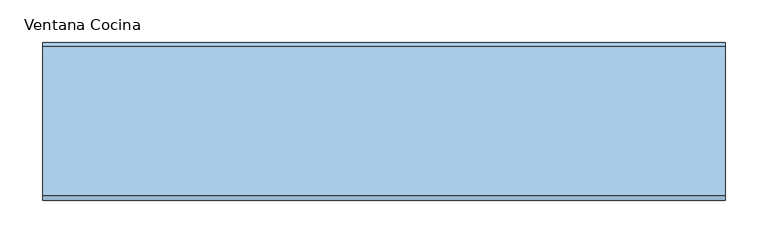
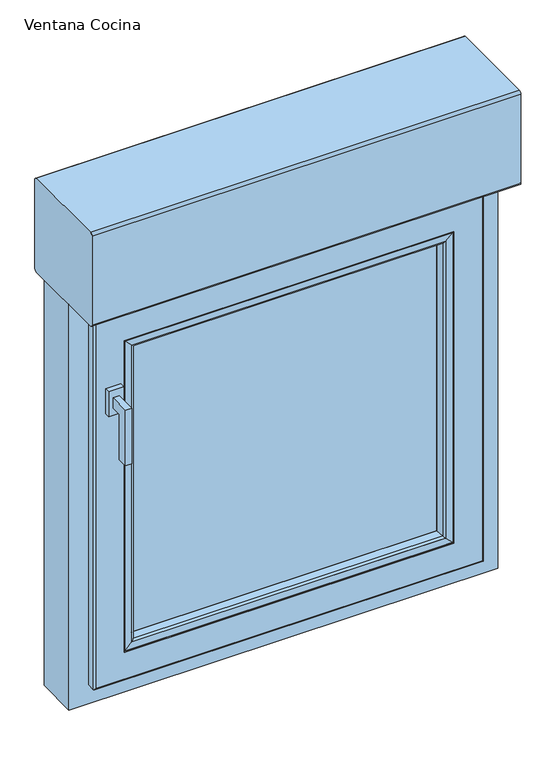
"""IFC4 building model written with IfcOpenShell, lengths in millimetres: window geometry, 2019_ES_Ventana_Replus_re80pvc301_10100_box_1-Hoja_con-Compacto : Ventana Cocina."""

from ifc_helpers import new_model, si_unit, point, frame, frame_2d, origin, place, context, project, spatial, polyline, circle_curve, ellipse_curve, trimmed, segment, composite_curve, outline, extrude, source, transform, mapped, element, save
from ifc_brep_helpers import plane_surface, cylinder_surface, advanced_brep


def ventana_cocina_321dc98e(model_context):
    return source(origin(), model_context, "Body", "SolidModel", [
        extrude(outline(composite_curve([segment(polyline([(55.0, 1610.0), (-120.0, 1610.0)]), True, "CONTINUOUS"), segment(trimmed(circle_curve(frame_2d((-120.0, 1615.0)), 5.0), [point((-120.0, 1610.0))], [point((-125.0, 1615.0))], False, "CARTESIAN"), True, "CONTINUOUS"), segment(polyline([(-125.0, 1615.0), (-125.0, 1790.0)]), True, "CONTINUOUS"), segment(trimmed(circle_curve(frame_2d((-120.0, 1790.0)), 5.0), [point((-125.0, 1790.0))], [point((-120.0, 1795.0))], False, "CARTESIAN"), True, "CONTINUOUS"), segment(polyline([(-120.0, 1795.0), (55.0, 1795.0)]), True, "CONTINUOUS"), segment(trimmed(circle_curve(frame_2d((55.0, 1790.0)), 5.0), [point((55.0, 1795.0))], [point((60.0, 1790.0))], False, "CARTESIAN"), True, "CONTINUOUS"), segment(polyline([(60.0, 1790.0), (60.0, 1615.0)]), True, "CONTINUOUS"), segment(trimmed(circle_curve(frame_2d((55.0, 1615.0)), 5.0), [point((60.0, 1615.0))], [point((55.0, 1610.0))], False, "CARTESIAN"), True, "CONTINUOUS")], self_intersect=False)), frame((-400.0, 0.0, 0.0), z_axis=(1.0, 0.0, 0.0), x_axis=(0.0, 1.0, 0.0)), (0.0, 0.0, 1.0), 800.0),
        extrude(outline(polyline([(-78.4999991, 1420.0), (-78.4999991, 1400.0), (-98.4999991, 1400.0), (-98.4999991, 1310.0), (-118.4999991, 1310.0), (-118.4999991, 1420.0), (-78.4999991, 1420.0)])), frame((-334.1999993, 0.0, 0.0), z_axis=(1.0, 0.0, 0.0), x_axis=(0.0, 1.0, 0.0)), (0.0, 0.0, 1.0), 12.0),
        extrude(outline(polyline([(-313.9687607, -78.4999991), (-342.4312378, -78.4999991), (-342.4312378, -68.4999991), (-313.9687607, -68.4999991), (-313.9687607, -78.4999991)])), frame((0.0, 0.0, 1385.217127), z_axis=(0.0, 0.0, 1.0), x_axis=(1.0, 0.0, 0.0)), (0.0, 0.0, 1.0), 49.565746),
        extrude(outline(polyline([(1507.2, 297.1999993), (1507.2, -297.1999993), (909.8, -297.1999993), (909.8, 297.1999993), (1507.2, 297.1999993)]), holes=[polyline([(917.8, 289.1999993), (917.8, -289.1999993), (1499.2, -289.1999993), (1499.2, 289.1999993), (917.8, 289.1999993)])]), frame((0.0, -26.9999999, 0.0), z_axis=(0.0, 1.0, 0.0), x_axis=(0.0, 0.0, 1.0)), (0.0, 0.0, 1.0), 16.0),
        extrude(outline(polyline([(1507.1868066, 297.1868058), (1507.1868066, -297.1868058), (909.8131934, -297.1868058), (909.8131934, 297.1868058), (1507.1868066, 297.1868058)]), holes=[polyline([(917.8, 289.1999993), (917.8, -289.1999993), (1499.2, -289.1999993), (1499.2, 289.1999993), (917.8, 289.1999993)])]), frame((0.0, -47.0000001, 0.0), z_axis=(0.0, 1.0, 0.0), x_axis=(0.0, 0.0, 1.0)), (0.0, 0.0, 1.0), 16.0),
        extrude(outline(polyline([(297.1999993, -6.9999997), (297.1999993, -10.9999999), (-297.1999993, -10.9999999), (-297.1999993, -6.9999997), (297.1999993, -6.9999997)])), frame((0.0, 0.0, 903.7946451), z_axis=(0.0, 0.0, 1.0), x_axis=(1.0, 0.0, 0.0)), (0.0, 0.0, 1.0), 609.4053549),
        extrude(outline(polyline([(297.1999993, -26.9999999), (297.1999993, -31.0000001), (-297.1999993, -31.0000001), (-297.1999993, -26.9999999), (297.1999993, -26.9999999)])), frame((0.0, 0.0, 903.7946451), z_axis=(0.0, 0.0, 1.0), x_axis=(1.0, 0.0, 0.0)), (0.0, 0.0, 1.0), 609.4053549),
        extrude(outline(polyline([(297.1999993, -47.0000001), (297.1999993, -51.0000003), (-297.1999993, -51.0000003), (-297.1999993, -47.0000001), (297.1999993, -47.0000001)])), frame((0.0, 0.0, 903.7946451), z_axis=(0.0, 0.0, 1.0), x_axis=(1.0, 0.0, 0.0)), (0.0, 0.0, 1.0), 609.4053549),
        advanced_brep(
        [(287.2913171, 9.2764571, 1497.2913178), (290.1890946, 11.5, 1500.1890953), (290.1890946, 11.5, 919.8109047), (287.2913171, 9.2764571, 922.7086822), (330.1999993, 11.5, 879.8), (-330.1999993, 11.5, 879.8), (-330.1999993, 11.5, 1540.2), (330.1999993, 11.5, 1540.2), (-290.1890946, 11.5, 1500.1890953), (-290.1890946, 11.5, 919.8109047), (-287.2913171, 9.2764571, 922.7086822), (284.1757968, -2.3508228, 1494.1757976), (284.1757968, -2.3508228, 925.8242024), (-284.1757968, -2.3508228, 925.8242024), (284.6739305, -3.0000033, 1494.6739313), (284.6739305, -3.0000033, 925.3260687), (-284.6739305, -3.0000033, 925.3260687), (291.1999993, -3.0000033, 1501.2), (-291.1999993, -3.0000033, 1501.2), (-291.1999993, -3.0000033, 918.8), (291.1999993, -3.0000033, 918.8), (-284.6739305, -3.0000033, 1494.6739313), (291.1999993, -6.9999997, 1501.2), (291.1999993, -6.9999997, 918.8), (-291.1999993, -6.9999997, 918.8), (311.8162192, -6.9999997, 1521.8162199), (-311.8162192, -6.9999997, 1521.8162199), (-311.8162192, -6.9999997, 898.1837801), (311.8162192, -6.9999997, 898.1837801), (-291.1999993, -6.9999997, 1501.2), (309.1999993, -25.6153717, 1519.2), (309.1999993, -25.6153717, 900.8), (-309.1999993, -25.6153717, 900.8), (309.1999993, -56.4999995, 1519.2), (309.1999993, -56.4999995, 900.8), (-309.1999993, -56.4999995, 900.8), (-309.1999993, -56.4999995, 1519.2), (297.1999993, -56.4999995, 1507.2), (-297.1999993, -56.4999995, 1507.2), (-297.1999993, -56.4999995, 912.8), (297.1999993, -56.4999995, 912.8), (297.1999993, -51.0000003, 1507.2), (297.1999993, -51.0000003, 912.8), (-297.1999993, -51.0000003, 912.8), (-297.1999993, -51.0000003, 1507.2), (286.007687, -51.0000003, 1496.0076877), (-286.007687, -51.0000003, 1496.0076877), (-286.007687, -51.0000003, 923.9923123), (286.007687, -51.0000003, 923.9923123), (285.4940999, -51.6693201, 1495.4941006), (285.4940999, -51.6693201, 924.5058994), (-285.4940999, -51.6693201, 924.5058994), (288.8993918, -64.3780426, 1498.8993925), (288.8993918, -64.3780426, 921.1006075), (-288.8993918, -64.3780426, 921.1006075), (292.6234971, -67.3403297, 1502.6234978), (292.6234971, -67.3403297, 917.3765022), (-292.6234971, -67.3403297, 917.3765022), (305.6488427, -67.7951848, 1515.6488434), (305.6488427, -67.7951848, 904.3511566), (-305.6488427, -67.7951848, 904.3511566), (306.1999993, -67.2629391, 1516.2), (306.1999993, -67.2629391, 903.8), (-306.1999993, -67.2629391, 903.8), (307.4370593, -68.4999991, 1517.43706), (307.4370593, -68.4999991, 902.56294), (-307.4370593, -68.4999991, 902.56294), (360.1999993, -68.4999991, 1570.2), (-360.1999993, -68.4999991, 1570.2), (-360.1999993, -68.4999991, 849.8), (360.1999993, -68.4999991, 849.8), (-307.4370593, -68.4999991, 1517.43706), (363.1999993, -65.4999991, 1573.2), (363.1999993, -65.4999991, 846.8), (-363.1999993, -65.4999991, 846.8), (363.1999993, -50.0, 1573.2), (363.1999993, -50.0, 846.8), (-363.1999993, -50.0, 846.8), (-363.1999993, -50.0, 1573.2), (343.1999993, -50.0, 1553.2), (-343.1999993, -50.0, 1553.2), (-343.1999993, -50.0, 866.8), (343.1999993, -50.0, 866.8), (343.1999993, -11.9999991, 866.8), (343.1999993, -11.9999991, 1553.2), (-343.1999993, -11.9999991, 866.8), (-343.1999993, -11.9999991, 1553.2), (330.1999993, -11.9999991, 1540.2), (-330.1999993, -11.9999991, 1540.2), (-330.1999993, -11.9999991, 879.8), (330.1999993, -11.9999991, 879.8), (-287.2913171, 9.2764571, 1497.2913178), (-284.1757968, -2.3508228, 1494.1757976), (-309.1999993, -25.6153717, 1519.2), (-285.4940999, -51.6693201, 1495.4941006), (-288.8993918, -64.3780426, 1498.8993925), (-292.6234971, -67.3403297, 1502.6234978), (-305.6488427, -67.7951848, 1515.6488434), (-306.1999993, -67.2629391, 1516.2), (-363.1999993, -65.4999991, 1573.2)],
        [
            (0, 1, ellipse_curve(frame((290.1890946, 8.5, 1500.1890953), z_axis=(0.7071067811865475, 0.0, -0.7071067811865475), x_axis=(0.7071067811865474, 0.0, 0.7071067811865476)), 4.2426407, 3.0)),
            (1, 2),
            (2, 3, ellipse_curve(frame((290.1890946, 8.5, 919.8109047), z_axis=(0.7071067811865475, 0.0, 0.7071067811865475), x_axis=(-0.7071067811865474, 0.0, 0.7071067811865476)), 4.2426407, 3.0)),
            (3, 0),
            (4, 5),
            (5, 6),
            (6, 7),
            (7, 4),
            (1, 8),
            (8, 9),
            (9, 2),
            (9, 10, ellipse_curve(frame((-290.1890946, 8.5, 919.8109047), z_axis=(0.7071067811865475, 0.0, -0.7071067811865475), x_axis=(0.7071067811865476, 0.0, 0.7071067811865474)), 4.2426407, 3.0)),
            (10, 3),
            (11, 0),
            (3, 12),
            (12, 11),
            (10, 13),
            (13, 12),
            (14, 11, ellipse_curve(frame((284.6739305, -2.4842973, 1494.6739313), z_axis=(0.7071067811865475, 0.0, -0.7071067811865475), x_axis=(0.7071067811865474, 0.0, 0.7071067811865476)), 0.7293184, 0.515706)),
            (12, 15, ellipse_curve(frame((284.6739305, -2.4842973, 925.3260687), z_axis=(0.7071067811865475, 0.0, 0.7071067811865475), x_axis=(-0.7071067811865474, 0.0, 0.7071067811865476)), 0.7293184, 0.515706)),
            (15, 14),
            (13, 16, ellipse_curve(frame((-284.6739305, -2.4842973, 925.3260687), z_axis=(0.7071067811865475, 0.0, -0.7071067811865475), x_axis=(0.7071067811865476, 0.0, 0.7071067811865474)), 0.7293184, 0.515706)),
            (16, 15),
            (17, 18),
            (18, 19),
            (19, 20),
            (20, 17),
            (16, 21),
            (21, 14),
            (22, 17),
            (20, 23),
            (23, 22),
            (19, 24),
            (24, 23),
            (25, 26),
            (26, 27),
            (27, 28),
            (28, 25),
            (24, 29),
            (29, 22),
            (30, 25),
            (28, 31),
            (31, 30),
            (27, 32),
            (32, 31),
            (33, 30),
            (31, 34),
            (34, 33),
            (32, 35),
            (35, 34),
            (35, 36),
            (36, 33),
            (37, 38),
            (38, 39),
            (39, 40),
            (40, 37),
            (41, 37),
            (40, 42),
            (42, 41),
            (39, 43),
            (43, 42),
            (43, 44),
            (44, 41),
            (45, 46),
            (46, 47),
            (47, 48),
            (48, 45),
            (49, 45, ellipse_curve(frame((286.007687, -51.5317048, 1496.0076877), z_axis=(0.7071067811865475, 0.0, -0.7071067811865475), x_axis=(0.7071067811865474, 0.0, 0.7071067811865476)), 0.7519437, 0.5317045)),
            (48, 50, ellipse_curve(frame((286.007687, -51.5317048, 923.9923123), z_axis=(0.7071067811865475, 0.0, 0.7071067811865475), x_axis=(-0.7071067811865474, 0.0, 0.7071067811865476)), 0.7519437, 0.5317045)),
            (50, 49),
            (47, 51, ellipse_curve(frame((-286.007687, -51.5317048, 923.9923123), z_axis=(0.7071067811865475, 0.0, -0.7071067811865475), x_axis=(0.7071067811865476, 0.0, 0.7071067811865474)), 0.7519437, 0.5317045)),
            (51, 50),
            (52, 49),
            (50, 53),
            (53, 52),
            (51, 54),
            (54, 53),
            (55, 52, ellipse_curve(frame((292.7630951, -63.3427664, 1502.7630958), z_axis=(0.7071067811865475, 0.0, -0.7071067811865475), x_axis=(0.7071067811865474, 0.0, 0.7071067811865476)), 5.6568542, 4.0)),
            (53, 56, ellipse_curve(frame((292.7630951, -63.3427664, 917.2369042), z_axis=(0.7071067811865475, 0.0, 0.7071067811865475), x_axis=(-0.7071067811865474, 0.0, 0.7071067811865476)), 5.6568542, 4.0)),
            (56, 55),
            (54, 57, ellipse_curve(frame((-292.7630951, -63.3427664, 917.2369042), z_axis=(0.7071067811865475, 0.0, -0.7071067811865475), x_axis=(0.7071067811865476, 0.0, 0.7071067811865474)), 5.6568542, 4.0)),
            (57, 56),
            (58, 55),
            (56, 59),
            (59, 58),
            (57, 60),
            (60, 59),
            (61, 58, ellipse_curve(frame((305.6674291, -67.2629391, 1515.6674299), z_axis=(0.7071067811865475, 0.0, -0.7071067811865475), x_axis=(0.7071067811865474, 0.0, 0.7071067811865476)), 0.7531679, 0.5325701)),
            (59, 62, ellipse_curve(frame((305.6674291, -67.2629391, 904.3325701), z_axis=(0.7071067811865475, 0.0, 0.7071067811865475), x_axis=(-0.7071067811865474, 0.0, 0.7071067811865476)), 0.7531679, 0.5325701)),
            (62, 61),
            (60, 63, ellipse_curve(frame((-305.6674291, -67.2629391, 904.3325701), z_axis=(0.7071067811865475, 0.0, -0.7071067811865475), x_axis=(0.7071067811865476, 0.0, 0.7071067811865474)), 0.7531679, 0.5325701)),
            (63, 62),
            (64, 61, ellipse_curve(frame((307.4370593, -67.2629391, 1517.43706), z_axis=(0.7071067811865475, 0.0, -0.7071067811865475), x_axis=(0.7071067811865474, 0.0, 0.7071067811865476)), 1.7494671, 1.23706)),
            (62, 65, ellipse_curve(frame((307.4370593, -67.2629391, 902.56294), z_axis=(0.7071067811865475, 0.0, 0.7071067811865475), x_axis=(-0.7071067811865474, 0.0, 0.7071067811865476)), 1.7494671, 1.23706)),
            (65, 64),
            (63, 66, ellipse_curve(frame((-307.4370593, -67.2629391, 902.56294), z_axis=(0.7071067811865475, 0.0, -0.7071067811865475), x_axis=(0.7071067811865476, 0.0, 0.7071067811865474)), 1.7494671, 1.23706)),
            (66, 65),
            (67, 68),
            (68, 69),
            (69, 70),
            (70, 67),
            (66, 71),
            (71, 64),
            (72, 67, ellipse_curve(frame((360.1999993, -65.4999991, 1570.2), z_axis=(0.7071067811865475, 0.0, -0.7071067811865475), x_axis=(0.7071067811865474, 0.0, 0.7071067811865476)), 4.2426407, 3.0)),
            (70, 73, ellipse_curve(frame((360.1999993, -65.4999991, 849.8), z_axis=(0.7071067811865475, 0.0, 0.7071067811865475), x_axis=(-0.7071067811865474, 0.0, 0.7071067811865476)), 4.2426407, 3.0)),
            (73, 72),
            (69, 74, ellipse_curve(frame((-360.1999993, -65.4999991, 849.8), z_axis=(0.7071067811865475, 0.0, -0.7071067811865475), x_axis=(0.7071067811865476, 0.0, 0.7071067811865474)), 4.2426407, 3.0)),
            (74, 73),
            (75, 72),
            (73, 76),
            (76, 75),
            (74, 77),
            (77, 76),
            (77, 78),
            (78, 75),
            (79, 80),
            (80, 81),
            (81, 82),
            (82, 79),
            (82, 83),
            (83, 84),
            (84, 79),
            (81, 85),
            (85, 83),
            (85, 86),
            (86, 84),
            (87, 88),
            (88, 89),
            (89, 90),
            (90, 87),
            (90, 4),
            (7, 87),
            (89, 5),
            (8, 91, ellipse_curve(frame((-290.1890946, 8.5, 1500.1890953), z_axis=(-0.7071067811865475, 0.0, -0.7071067811865475), x_axis=(0.7071067811865474, 0.0, -0.7071067811865476)), 4.2426407, 3.0)),
            (91, 10),
            (91, 92),
            (92, 13),
            (92, 21, ellipse_curve(frame((-284.6739305, -2.4842973, 1494.6739313), z_axis=(-0.7071067811865475, 0.0, -0.7071067811865475), x_axis=(0.7071067811865474, 0.0, -0.7071067811865476)), 0.7293184, 0.515706)),
            (18, 29),
            (26, 93),
            (93, 32),
            (93, 36),
            (38, 44),
            (46, 94, ellipse_curve(frame((-286.007687, -51.5317048, 1496.0076877), z_axis=(-0.7071067811865475, 0.0, -0.7071067811865475), x_axis=(0.7071067811865474, 0.0, -0.7071067811865476)), 0.7519437, 0.5317045)),
            (94, 51),
            (94, 95),
            (95, 54),
            (95, 96, ellipse_curve(frame((-292.7630951, -63.3427664, 1502.7630958), z_axis=(-0.7071067811865475, 0.0, -0.7071067811865475), x_axis=(0.7071067811865474, 0.0, -0.7071067811865476)), 5.6568542, 4.0)),
            (96, 57),
            (96, 97),
            (97, 60),
            (97, 98, ellipse_curve(frame((-305.6674291, -67.2629391, 1515.6674299), z_axis=(-0.7071067811865475, 0.0, -0.7071067811865475), x_axis=(0.7071067811865474, 0.0, -0.7071067811865476)), 0.7531679, 0.5325701)),
            (98, 63),
            (98, 71, ellipse_curve(frame((-307.4370593, -67.2629391, 1517.43706), z_axis=(-0.7071067811865475, 0.0, -0.7071067811865475), x_axis=(0.7071067811865474, 0.0, -0.7071067811865476)), 1.7494671, 1.23706)),
            (68, 99, ellipse_curve(frame((-360.1999993, -65.4999991, 1570.2), z_axis=(-0.7071067811865475, 0.0, -0.7071067811865475), x_axis=(0.7071067811865474, 0.0, -0.7071067811865476)), 4.2426407, 3.0)),
            (99, 74),
            (99, 78),
            (80, 86),
            (88, 6),
            (0, 91),
            (11, 92),
            (30, 93),
            (49, 94),
            (52, 95),
            (55, 96),
            (58, 97),
            (61, 98),
            (72, 99),
        ],
        [
            cylinder_surface(frame((290.1890946, 8.5, 1573.2), z_axis=(0.0, 0.0, 1.0), x_axis=(-1.0, 0.0, 0.0)), 3.0),
            plane_surface(frame((-330.1999993, 11.5, 1540.2), z_axis=(0.0, 1.0, 0.0), x_axis=(1.0, 0.0, 0.0))),
            cylinder_surface(frame((363.1999993, 8.5, 919.8109047), z_axis=(1.0, 0.0, 0.0), x_axis=(0.0, 0.0, 1.0)), 3.0),
            plane_surface(frame((287.2913171, 9.2764571, 1497.2913178), z_axis=(-0.9659258263570556, 0.258819044848789, 0.0), x_axis=(0.0, 0.0, -1.0))),
            plane_surface(frame((287.2913171, 9.2764571, 922.7086822), z_axis=(0.0, 0.2588190448487859, 0.9659258263570565), x_axis=(-1.0, 0.0, 0.0))),
            cylinder_surface(frame((284.6739305, -2.4842973, 1573.2), z_axis=(0.0, 0.0, 1.0), x_axis=(-1.0, 0.0, 0.0)), 0.515706),
            cylinder_surface(frame((363.1999993, -2.4842973, 925.3260687), z_axis=(1.0, 0.0, 0.0), x_axis=(0.0, 0.0, 1.0)), 0.515706),
            plane_surface(frame((-284.6739305, -3.0000033, 1494.6739313), z_axis=(0.0, -1.0, 0.0), x_axis=(1.0, 0.0, 0.0))),
            plane_surface(frame((291.1999993, -3.0000033, 1501.2), z_axis=(-1.0, 0.0, 0.0), x_axis=(0.0, 0.0, -1.0))),
            plane_surface(frame((291.1999993, -3.0000033, 918.8), z_axis=(0.0, 0.0, 1.0), x_axis=(-1.0, 0.0, 0.0))),
            plane_surface(frame((-291.1999993, -6.9999997, 1501.2), z_axis=(0.0, -1.0, 0.0), x_axis=(1.0, 0.0, 0.0))),
            plane_surface(frame((311.8162192, -6.9999997, 1521.8162199), z_axis=(-0.9902680687415736, 0.13917310096004265, 0.0), x_axis=(0.0, 0.0, -1.0))),
            plane_surface(frame((311.8162192, -6.9999997, 898.1837801), z_axis=(0.0, 0.13917310096003943, 0.990268068741574), x_axis=(-1.0, 0.0, 0.0))),
            plane_surface(frame((309.1999993, -25.6153717, 1519.2), z_axis=(-1.0, 0.0, 0.0), x_axis=(0.0, 0.0, -1.0))),
            plane_surface(frame((309.1999993, -25.6153717, 900.8), z_axis=(0.0, 0.0, 1.0), x_axis=(-1.0, 0.0, 0.0))),
            plane_surface(frame((-309.1999993, -56.4999995, 1519.2), z_axis=(0.0, 1.0, 0.0), x_axis=(1.0, 0.0, 0.0))),
            plane_surface(frame((297.1999993, -56.4999995, 1507.2), z_axis=(1.0, 0.0, 0.0), x_axis=(0.0, 0.0, -1.0))),
            plane_surface(frame((297.1999993, -56.4999995, 912.8), z_axis=(0.0, 0.0, -1.0), x_axis=(-1.0, 0.0, 0.0))),
            plane_surface(frame((-297.1999993, -51.0000003, 1507.2), z_axis=(0.0, 1.0, 0.0), x_axis=(1.0, 0.0, 0.0))),
            cylinder_surface(frame((286.007687, -51.5317048, 1573.2), z_axis=(0.0, 0.0, 1.0), x_axis=(-1.0, 0.0, 0.0)), 0.5317045),
            cylinder_surface(frame((363.1999993, -51.5317048, 923.9923123), z_axis=(1.0, 0.0, 0.0), x_axis=(0.0, 0.0, 1.0)), 0.5317045),
            plane_surface(frame((285.4940999, -51.6693201, 1495.4941006), z_axis=(-0.9659258262890666, -0.2588190451025272, 0.0), x_axis=(0.0, 0.0, -1.0))),
            plane_surface(frame((285.4940999, -51.6693201, 924.5058994), z_axis=(0.0, -0.2588190451025303, 0.9659258262890658), x_axis=(-1.0, 0.0, 0.0))),
            cylinder_surface(frame((292.7630951, -63.3427664, 1573.2), z_axis=(0.0, 0.0, 1.0), x_axis=(-1.0, 0.0, 0.0)), 4.0),
            cylinder_surface(frame((363.1999993, -63.3427664, 917.2369042), z_axis=(1.0, 0.0, 0.0), x_axis=(0.0, 0.0, 1.0)), 4.0),
            plane_surface(frame((292.6234971, -67.3403297, 1502.6234978), z_axis=(-0.03489949670250791, -0.9993908270190955, 0.0), x_axis=(0.0, 0.0, -1.0))),
            plane_surface(frame((292.6234971, -67.3403297, 917.3765022), z_axis=(0.0, -0.9993908270190957, 0.034899496702504675), x_axis=(-1.0, 0.0, 0.0))),
            cylinder_surface(frame((305.6674291, -67.2629391, 1573.2), z_axis=(0.0, 0.0, 1.0), x_axis=(-1.0, 0.0, 0.0)), 0.5325701),
            cylinder_surface(frame((363.1999993, -67.2629391, 904.3325701), z_axis=(1.0, 0.0, 0.0), x_axis=(0.0, 0.0, 1.0)), 0.5325701),
            cylinder_surface(frame((307.4370593, -67.2629391, 1573.2), z_axis=(0.0, 0.0, 1.0), x_axis=(-1.0, 0.0, 0.0)), 1.23706),
            cylinder_surface(frame((363.1999993, -67.2629391, 902.56294), z_axis=(1.0, 0.0, 0.0), x_axis=(0.0, 0.0, 1.0)), 1.23706),
            plane_surface(frame((-307.4370593, -68.4999991, 1517.43706), z_axis=(0.0, -1.0, 0.0), x_axis=(1.0, 0.0, 0.0))),
            cylinder_surface(frame((360.1999993, -65.4999991, 1573.2), z_axis=(0.0, 0.0, 1.0), x_axis=(-1.0, 0.0, 0.0)), 3.0),
            cylinder_surface(frame((363.1999993, -65.4999991, 849.8), z_axis=(1.0, 0.0, 0.0), x_axis=(0.0, 0.0, 1.0)), 3.0),
            plane_surface(frame((363.1999993, -65.4999991, 1573.2), z_axis=(1.0, 0.0, 0.0), x_axis=(0.0, 0.0, -1.0))),
            plane_surface(frame((363.1999993, -65.4999991, 846.8), z_axis=(0.0, 0.0, -1.0), x_axis=(-1.0, 0.0, 0.0))),
            plane_surface(frame((-359.2000019, -50.0, 1569.2000027), z_axis=(0.0, 1.0, 0.0), x_axis=(1.0, 0.0, 0.0))),
            plane_surface(frame((343.1999993, -45.0999991, 1553.2), z_axis=(1.0, 0.0, 0.0), x_axis=(0.0, 0.0, -1.0))),
            plane_surface(frame((343.1999993, -45.0999991, 866.8), z_axis=(0.0, 0.0, -1.0), x_axis=(-1.0, 0.0, 0.0))),
            plane_surface(frame((-335.7000002, -11.9999991, 1545.7000009), z_axis=(0.0, 1.0, 0.0), x_axis=(1.0, 0.0, 0.0))),
            plane_surface(frame((330.1999993, -1.4999991, 1540.2), z_axis=(1.0, 0.0, 0.0), x_axis=(0.0, 0.0, -1.0))),
            plane_surface(frame((330.1999993, -1.4999991, 879.8), z_axis=(0.0, 0.0, -1.0), x_axis=(-1.0, 0.0, 0.0))),
            cylinder_surface(frame((-290.1890946, 8.5, 846.8), z_axis=(0.0, 0.0, -1.0), x_axis=(1.0, 0.0, 0.0)), 3.0),
            plane_surface(frame((-287.2913171, 9.2764571, 922.7086822), z_axis=(0.9659258263570573, 0.25881904484878276, 0.0), x_axis=(0.0, 0.0, 1.0))),
            cylinder_surface(frame((-284.6739305, -2.4842973, 846.8), z_axis=(0.0, 0.0, -1.0), x_axis=(1.0, 0.0, 0.0)), 0.515706),
            plane_surface(frame((-291.1999993, -3.0000033, 918.8), z_axis=(1.0, 0.0, 0.0), x_axis=(0.0, 0.0, 1.0))),
            plane_surface(frame((-311.8162192, -6.9999997, 898.1837801), z_axis=(0.9902680687415745, 0.1391731009600362, 0.0), x_axis=(0.0, 0.0, 1.0))),
            plane_surface(frame((-309.1999993, -25.6153717, 900.8), z_axis=(1.0, 0.0, 0.0), x_axis=(0.0, 0.0, 1.0))),
            plane_surface(frame((-297.1999993, -56.4999995, 912.8), z_axis=(-1.0, 0.0, 0.0), x_axis=(0.0, 0.0, 1.0))),
            cylinder_surface(frame((-286.007687, -51.5317048, 846.8), z_axis=(0.0, 0.0, -1.0), x_axis=(1.0, 0.0, 0.0)), 0.5317045),
            plane_surface(frame((-285.4940999, -51.6693201, 924.5058994), z_axis=(0.9659258262890649, -0.2588190451025334, 0.0), x_axis=(0.0, 0.0, 1.0))),
            cylinder_surface(frame((-292.7630951, -63.3427664, 846.8), z_axis=(0.0, 0.0, -1.0), x_axis=(1.0, 0.0, 0.0)), 4.0),
            plane_surface(frame((-292.6234971, -67.3403297, 917.3765022), z_axis=(0.03489949670250144, -0.9993908270190958, 0.0), x_axis=(0.0, 0.0, 1.0))),
            cylinder_surface(frame((-305.6674291, -67.2629391, 846.8), z_axis=(0.0, 0.0, -1.0), x_axis=(1.0, 0.0, 0.0)), 0.5325701),
            cylinder_surface(frame((-307.4370593, -67.2629391, 846.8), z_axis=(0.0, 0.0, -1.0), x_axis=(1.0, 0.0, 0.0)), 1.23706),
            cylinder_surface(frame((-360.1999993, -65.4999991, 846.8), z_axis=(0.0, 0.0, -1.0), x_axis=(1.0, 0.0, 0.0)), 3.0),
            plane_surface(frame((-363.1999993, -65.4999991, 846.8), z_axis=(-1.0, 0.0, 0.0), x_axis=(0.0, 0.0, 1.0))),
            plane_surface(frame((-343.1999993, -45.0999991, 866.8), z_axis=(-1.0, 0.0, 0.0), x_axis=(0.0, 0.0, 1.0))),
            plane_surface(frame((-330.1999993, -1.4999991, 879.8), z_axis=(-1.0, 0.0, 0.0), x_axis=(0.0, 0.0, 1.0))),
            cylinder_surface(frame((-363.1999993, 8.5, 1500.1890953), z_axis=(-1.0, 0.0, 0.0), x_axis=(0.0, 0.0, -1.0)), 3.0),
            plane_surface(frame((-287.2913171, 9.2764571, 1497.2913178), z_axis=(0.0, 0.2588190448487859, -0.9659258263570564), x_axis=(1.0, 0.0, 0.0))),
            cylinder_surface(frame((-363.1999993, -2.4842973, 1494.6739313), z_axis=(-1.0, 0.0, 0.0), x_axis=(0.0, 0.0, -1.0)), 0.515706),
            plane_surface(frame((-291.1999993, -3.0000033, 1501.2), z_axis=(0.0, 0.0, -1.0), x_axis=(1.0, 0.0, 0.0))),
            plane_surface(frame((-311.8162192, -6.9999997, 1521.8162199), z_axis=(0.0, 0.13917310096003943, -0.990268068741574), x_axis=(1.0, 0.0, 0.0))),
            plane_surface(frame((-309.1999993, -25.6153717, 1519.2), z_axis=(0.0, 0.0, -1.0), x_axis=(1.0, 0.0, 0.0))),
            plane_surface(frame((-297.1999993, -56.4999995, 1507.2), z_axis=(0.0, 0.0, 1.0), x_axis=(1.0, 0.0, 0.0))),
            cylinder_surface(frame((-363.1999993, -51.5317048, 1496.0076877), z_axis=(-1.0, 0.0, 0.0), x_axis=(0.0, 0.0, -1.0)), 0.5317045),
            plane_surface(frame((-285.4940999, -51.6693201, 1495.4941006), z_axis=(0.0, -0.2588190451025303, -0.9659258262890658), x_axis=(1.0, 0.0, 0.0))),
            cylinder_surface(frame((-363.1999993, -63.3427664, 1502.7630958), z_axis=(-1.0, 0.0, 0.0), x_axis=(0.0, 0.0, -1.0)), 4.0),
            plane_surface(frame((-292.6234971, -67.3403297, 1502.6234978), z_axis=(0.0, -0.9993908270190957, -0.034899496702504675), x_axis=(1.0, 0.0, 0.0))),
            cylinder_surface(frame((-363.1999993, -67.2629391, 1515.6674299), z_axis=(-1.0, 0.0, 0.0), x_axis=(0.0, 0.0, -1.0)), 0.5325701),
            cylinder_surface(frame((-363.1999993, -67.2629391, 1517.43706), z_axis=(-1.0, 0.0, 0.0), x_axis=(0.0, 0.0, -1.0)), 1.23706),
            cylinder_surface(frame((-363.1999993, -65.4999991, 1570.2), z_axis=(-1.0, 0.0, 0.0), x_axis=(0.0, 0.0, -1.0)), 3.0),
            plane_surface(frame((-363.1999993, -65.4999991, 1573.2), z_axis=(0.0, 0.0, 1.0), x_axis=(1.0, 0.0, 0.0))),
            plane_surface(frame((-343.1999993, -45.0999991, 1553.2), z_axis=(0.0, 0.0, 1.0), x_axis=(1.0, 0.0, 0.0))),
            plane_surface(frame((-330.1999993, -1.4999991, 1540.2), z_axis=(0.0, 0.0, 1.0), x_axis=(1.0, 0.0, 0.0))),
        ],
        [
            (0, [[1, 2, 3, 4]]),
            (1, [[5, 6, 7, 8], [9, 10, 11, -2]]),
            (2, [[-3, -11, 12, 13]]),
            (3, [[14, -4, 15, 16]]),
            (4, [[-15, -13, 17, 18]]),
            (5, [[19, -16, 20, 21]]),
            (6, [[-20, -18, 22, 23]]),
            (7, [[24, 25, 26, 27], [-23, 28, 29, -21]]),
            (8, [[30, -27, 31, 32]]),
            (9, [[-31, -26, 33, 34]]),
            (10, [[35, 36, 37, 38], [-34, 39, 40, -32]]),
            (11, [[41, -38, 42, 43]]),
            (12, [[-42, -37, 44, 45]]),
            (13, [[46, -43, 47, 48]]),
            (14, [[-47, -45, 49, 50]]),
            (15, [[-50, 51, 52, -48], [53, 54, 55, 56]]),
            (16, [[57, -56, 58, 59]]),
            (17, [[-58, -55, 60, 61]]),
            (18, [[-61, 62, 63, -59], [64, 65, 66, 67]]),
            (19, [[68, -67, 69, 70]]),
            (20, [[-69, -66, 71, 72]]),
            (21, [[73, -70, 74, 75]]),
            (22, [[-74, -72, 76, 77]]),
            (23, [[78, -75, 79, 80]]),
            (24, [[-79, -77, 81, 82]]),
            (25, [[83, -80, 84, 85]]),
            (26, [[-84, -82, 86, 87]]),
            (27, [[88, -85, 89, 90]]),
            (28, [[-89, -87, 91, 92]]),
            (29, [[93, -90, 94, 95]]),
            (30, [[-94, -92, 96, 97]]),
            (31, [[98, 99, 100, 101], [-97, 102, 103, -95]]),
            (32, [[104, -101, 105, 106]]),
            (33, [[-105, -100, 107, 108]]),
            (34, [[109, -106, 110, 111]]),
            (35, [[-110, -108, 112, 113]]),
            (36, [[-113, 114, 115, -111], [116, 117, 118, 119]]),
            (37, [[-119, 120, 121, 122]]),
            (38, [[-120, -118, 123, 124]]),
            (39, [[-124, 125, 126, -121], [127, 128, 129, 130]]),
            (40, [[-130, 131, -8, 132]]),
            (41, [[-131, -129, 133, -5]]),
            (42, [[-12, -10, 134, 135]]),
            (43, [[-17, -135, 136, 137]]),
            (44, [[-22, -137, 138, -28]]),
            (45, [[-33, -25, 139, -39]]),
            (46, [[-44, -36, 140, 141]]),
            (47, [[-49, -141, 142, -51]]),
            (48, [[-60, -54, 143, -62]]),
            (49, [[-71, -65, 144, 145]]),
            (50, [[-76, -145, 146, 147]]),
            (51, [[-81, -147, 148, 149]]),
            (52, [[-86, -149, 150, 151]]),
            (53, [[-91, -151, 152, 153]]),
            (54, [[-96, -153, 154, -102]]),
            (55, [[-107, -99, 155, 156]]),
            (56, [[-112, -156, 157, -114]]),
            (57, [[-123, -117, 158, -125]]),
            (58, [[-133, -128, 159, -6]]),
            (59, [[-134, -9, -1, 160]]),
            (60, [[-136, -160, -14, 161]]),
            (61, [[-138, -161, -19, -29]]),
            (62, [[-139, -24, -30, -40]]),
            (63, [[-140, -35, -41, 162]]),
            (64, [[-142, -162, -46, -52]]),
            (65, [[-143, -53, -57, -63]]),
            (66, [[-144, -64, -68, 163]]),
            (67, [[-146, -163, -73, 164]]),
            (68, [[-148, -164, -78, 165]]),
            (69, [[-150, -165, -83, 166]]),
            (70, [[-152, -166, -88, 167]]),
            (71, [[-154, -167, -93, -103]]),
            (72, [[-155, -98, -104, 168]]),
            (73, [[-157, -168, -109, -115]]),
            (74, [[-158, -116, -122, -126]]),
            (75, [[-159, -127, -132, -7]]),
        ],
    ),
        advanced_brep(
        [(323.2673545, 12.758819, 1533.2673545), (327.2913185, 27.7764571, 1537.2913185), (327.2913185, 27.7764571, 882.7086815), (323.2673545, 12.758819, 886.7326455), (330.189096, 30.0, 1540.189096), (330.189096, 30.0, 879.810904), (-327.2913185, 27.7764571, 882.7086815), (-323.2673545, 12.758819, 886.7326455), (324.2332803, 11.5, 1534.2332803), (324.2332803, 11.5, 885.7667197), (400.0, 30.0, 1610.0), (400.0, -50.0, 1610.0), (400.0, -50.0, 810.0), (400.0, 30.0, 810.0), (-400.0, -50.0, 1610.0), (-400.0, -50.0, 810.0), (356.1999993, -50.0, 853.8000007), (-356.1999993, -50.0, 853.8000007), (-356.1999993, -50.0, 1566.1999993), (356.1999993, -50.0, 1566.1999993), (-400.0, 30.0, 810.0), (-400.0, 30.0, 1610.0), (-330.189096, 30.0, 1540.189096), (-330.189096, 30.0, 879.810904), (336.1891471, -8.0, 1546.1891471), (336.1891471, 11.5, 1546.1891471), (336.1891471, 11.5, 873.8108529), (336.1891471, -8.0, 873.8108529), (-336.1891471, 11.5, 1546.1891471), (-336.1891471, 11.5, 873.8108529), (-324.2332803, 11.5, 885.7667197), (-324.2332803, 11.5, 1534.2332803), (-336.1891471, -8.0, 873.8108529), (355.1999993, -8.0, 1565.1999993), (-355.1999993, -8.0, 1565.1999993), (-355.1999993, -8.0, 854.8000007), (355.1999993, -8.0, 854.8000007), (-336.1891471, -8.0, 1546.1891471), (355.1999993, -49.0, 1565.1999993), (355.1999993, -49.0, 854.8000007), (-355.1999993, -49.0, 854.8000007), (-327.2913185, 27.7764571, 1537.2913185), (-323.2673545, 12.758819, 1533.2673545), (-355.1999993, -49.0, 1565.1999993)],
        [
            (0, 1),
            (1, 2),
            (2, 3),
            (3, 0),
            (1, 4, ellipse_curve(frame((330.189096, 27.0, 1540.189096), z_axis=(0.7071067811865475, 0.0, -0.7071067811865475), x_axis=(0.7071067811865474, 0.0, 0.7071067811865476)), 4.2426407, 3.0)),
            (4, 5),
            (5, 2, ellipse_curve(frame((330.189096, 27.0, 879.810904), z_axis=(0.7071067811865475, 0.0, 0.7071067811865475), x_axis=(-0.7071067811865474, 0.0, 0.7071067811865476)), 4.2426407, 3.0)),
            (2, 6),
            (6, 7),
            (7, 3),
            (8, 0, ellipse_curve(frame((324.2332803, 12.5, 1534.2332803), z_axis=(0.7071067811865475, 0.0, -0.7071067811865475), x_axis=(0.7071067811865474, 0.0, 0.7071067811865476)), 1.4142136, 1.0)),
            (3, 9, ellipse_curve(frame((324.2332803, 12.5, 885.7667197), z_axis=(0.7071067811865475, 0.0, 0.7071067811865475), x_axis=(-0.7071067811865474, 0.0, 0.7071067811865476)), 1.4142136, 1.0)),
            (9, 8),
            (10, 11),
            (11, 12),
            (12, 13),
            (13, 10),
            (11, 14),
            (14, 15),
            (15, 12),
            (16, 17),
            (17, 18),
            (18, 19),
            (19, 16),
            (15, 20),
            (20, 13),
            (20, 21),
            (21, 10),
            (4, 22),
            (22, 23),
            (23, 5),
            (24, 25),
            (25, 26),
            (26, 27),
            (27, 24),
            (25, 28),
            (28, 29),
            (29, 26),
            (9, 30),
            (30, 31),
            (31, 8),
            (29, 32),
            (32, 27),
            (33, 34),
            (34, 35),
            (35, 36),
            (36, 33),
            (32, 37),
            (37, 24),
            (19, 38, ellipse_curve(frame((356.1999993, -49.0, 1566.1999993), z_axis=(0.7071067811865475, 0.0, -0.7071067811865475), x_axis=(0.7071067811865474, 0.0, 0.7071067811865476)), 1.4142136, 1.0)),
            (38, 39),
            (39, 16, ellipse_curve(frame((356.1999993, -49.0, 853.8000007), z_axis=(0.7071067811865475, 0.0, 0.7071067811865475), x_axis=(-0.7071067811865474, 0.0, 0.7071067811865476)), 1.4142136, 1.0)),
            (38, 33),
            (36, 39),
            (39, 40),
            (40, 17, ellipse_curve(frame((-356.1999993, -49.0, 853.8000007), z_axis=(0.7071067811865475, 0.0, -0.7071067811865475), x_axis=(0.7071067811865476, 0.0, 0.7071067811865474)), 1.4142136, 1.0)),
            (7, 30, ellipse_curve(frame((-324.2332803, 12.5, 885.7667197), z_axis=(0.7071067811865475, 0.0, -0.7071067811865475), x_axis=(0.7071067811865476, 0.0, 0.7071067811865474)), 1.4142136, 1.0)),
            (23, 6, ellipse_curve(frame((-330.189096, 27.0, 879.810904), z_axis=(0.7071067811865475, 0.0, -0.7071067811865475), x_axis=(0.7071067811865476, 0.0, 0.7071067811865474)), 4.2426407, 3.0)),
            (6, 41),
            (41, 42),
            (42, 7),
            (14, 21),
            (28, 37),
            (35, 40),
            (40, 43),
            (43, 18, ellipse_curve(frame((-356.1999993, -49.0, 1566.1999993), z_axis=(-0.7071067811865475, 0.0, -0.7071067811865475), x_axis=(0.7071067811865474, 0.0, -0.7071067811865476)), 1.4142136, 1.0)),
            (42, 31, ellipse_curve(frame((-324.2332803, 12.5, 1534.2332803), z_axis=(-0.7071067811865475, 0.0, -0.7071067811865475), x_axis=(0.7071067811865474, 0.0, -0.7071067811865476)), 1.4142136, 1.0)),
            (22, 41, ellipse_curve(frame((-330.189096, 27.0, 1540.189096), z_axis=(-0.7071067811865475, 0.0, -0.7071067811865475), x_axis=(0.7071067811865474, 0.0, -0.7071067811865476)), 4.2426407, 3.0)),
            (34, 43),
            (41, 1),
            (0, 42),
            (43, 38),
        ],
        [
            plane_surface(frame((327.2913185, 27.7764571, 1537.2913185), z_axis=(-0.9659258262890693, 0.25881904510251696, 0.0), x_axis=(0.0, 0.0, -1.0))),
            cylinder_surface(frame((330.189096, 27.0, 1610.0), z_axis=(0.0, 0.0, 1.0), x_axis=(-1.0, 0.0, 0.0)), 3.0),
            plane_surface(frame((327.2913185, 27.7764571, 882.7086815), z_axis=(0.0, 0.25881904510251386, 0.9659258262890702), x_axis=(-1.0, 0.0, 0.0))),
            cylinder_surface(frame((324.2332803, 12.5, 1610.0), z_axis=(0.0, 0.0, 1.0), x_axis=(-1.0, 0.0, 0.0)), 1.0),
            plane_surface(frame((400.0, -50.0, 1610.0), z_axis=(1.0, 0.0, 0.0), x_axis=(0.0, 0.0, -1.0))),
            plane_surface(frame((-356.1999993, -50.0, 1566.1999993), z_axis=(0.0, -1.0, 0.0), x_axis=(1.0, 0.0, 0.0))),
            plane_surface(frame((400.0, -50.0, 810.0), z_axis=(0.0, 0.0, -1.0), x_axis=(-1.0, 0.0, 0.0))),
            plane_surface(frame((-400.0, 30.0, 1610.0), z_axis=(0.0, 1.0, 0.0), x_axis=(1.0, 0.0, 0.0))),
            plane_surface(frame((336.1891471, 11.5, 1546.1891471), z_axis=(-1.0, 0.0, 0.0), x_axis=(0.0, 0.0, -1.0))),
            plane_surface(frame((-324.2332803, 11.5, 1534.2332803), z_axis=(0.0, -1.0, 0.0), x_axis=(1.0, 0.0, 0.0))),
            plane_surface(frame((336.1891471, 11.5, 873.8108529), z_axis=(0.0, 0.0, 1.0), x_axis=(-1.0, 0.0, 0.0))),
            plane_surface(frame((-336.1891471, -8.0, 1546.1891471), z_axis=(0.0, -1.0, 0.0), x_axis=(1.0, 0.0, 0.0))),
            cylinder_surface(frame((356.1999993, -49.0, 1610.0), z_axis=(0.0, 0.0, 1.0), x_axis=(-1.0, 0.0, 0.0)), 1.0),
            plane_surface(frame((355.1999993, -8.0, 1565.1999993), z_axis=(-1.0, 0.0, 0.0), x_axis=(0.0, 0.0, -1.0))),
            cylinder_surface(frame((400.0, -49.0, 853.8000007), z_axis=(1.0, 0.0, 0.0), x_axis=(0.0, 0.0, 1.0)), 1.0),
            cylinder_surface(frame((400.0, 12.5, 885.7667197), z_axis=(1.0, 0.0, 0.0), x_axis=(0.0, 0.0, 1.0)), 1.0),
            cylinder_surface(frame((400.0, 27.0, 879.810904), z_axis=(1.0, 0.0, 0.0), x_axis=(0.0, 0.0, 1.0)), 3.0),
            plane_surface(frame((-327.2913185, 27.7764571, 882.7086815), z_axis=(0.9659258262890711, 0.25881904510251075, 0.0), x_axis=(0.0, 0.0, 1.0))),
            plane_surface(frame((-400.0, -50.0, 810.0), z_axis=(-1.0, 0.0, 0.0), x_axis=(0.0, 0.0, 1.0))),
            plane_surface(frame((-336.1891471, 11.5, 873.8108529), z_axis=(1.0, 0.0, 0.0), x_axis=(0.0, 0.0, 1.0))),
            plane_surface(frame((355.1999993, -8.0, 854.8000007), z_axis=(0.0, 0.0, 1.0), x_axis=(-1.0, 0.0, 0.0))),
            cylinder_surface(frame((-356.1999993, -49.0, 810.0), z_axis=(0.0, 0.0, -1.0), x_axis=(1.0, 0.0, 0.0)), 1.0),
            cylinder_surface(frame((-324.2332803, 12.5, 810.0), z_axis=(0.0, 0.0, -1.0), x_axis=(1.0, 0.0, 0.0)), 1.0),
            cylinder_surface(frame((-330.189096, 27.0, 810.0), z_axis=(0.0, 0.0, -1.0), x_axis=(1.0, 0.0, 0.0)), 3.0),
            plane_surface(frame((-355.1999993, -8.0, 854.8000007), z_axis=(1.0, 0.0, 0.0), x_axis=(0.0, 0.0, 1.0))),
            plane_surface(frame((-327.2913185, 27.7764571, 1537.2913185), z_axis=(0.0, 0.25881904510251386, -0.9659258262890702), x_axis=(1.0, 0.0, 0.0))),
            plane_surface(frame((-400.0, -50.0, 1610.0), z_axis=(0.0, 0.0, 1.0), x_axis=(1.0, 0.0, 0.0))),
            plane_surface(frame((-336.1891471, 11.5, 1546.1891471), z_axis=(0.0, 0.0, -1.0), x_axis=(1.0, 0.0, 0.0))),
            cylinder_surface(frame((-400.0, -49.0, 1566.1999993), z_axis=(-1.0, 0.0, 0.0), x_axis=(0.0, 0.0, -1.0)), 1.0),
            cylinder_surface(frame((-400.0, 12.5, 1534.2332803), z_axis=(-1.0, 0.0, 0.0), x_axis=(0.0, 0.0, -1.0)), 1.0),
            cylinder_surface(frame((-400.0, 27.0, 1540.189096), z_axis=(-1.0, 0.0, 0.0), x_axis=(0.0, 0.0, -1.0)), 3.0),
            plane_surface(frame((-355.1999993, -8.0, 1565.1999993), z_axis=(0.0, 0.0, -1.0), x_axis=(1.0, 0.0, 0.0))),
        ],
        [
            (0, [[1, 2, 3, 4]]),
            (1, [[5, 6, 7, -2]]),
            (2, [[-3, 8, 9, 10]]),
            (3, [[11, -4, 12, 13]]),
            (4, [[14, 15, 16, 17]]),
            (5, [[18, 19, 20, -15], [21, 22, 23, 24]]),
            (6, [[-16, -20, 25, 26]]),
            (7, [[-26, 27, 28, -17], [29, 30, 31, -6]]),
            (8, [[32, 33, 34, 35]]),
            (9, [[36, 37, 38, -33], [39, 40, 41, -13]]),
            (10, [[-34, -38, 42, 43]]),
            (11, [[44, 45, 46, 47], [-43, 48, 49, -35]]),
            (12, [[50, 51, 52, -24]]),
            (13, [[53, -47, 54, -51]]),
            (14, [[-52, 55, 56, -21]]),
            (15, [[-12, -10, 57, -39]]),
            (16, [[-7, -31, 58, -8]]),
            (17, [[-9, 59, 60, 61]]),
            (18, [[-25, -19, 62, -27]]),
            (19, [[-42, -37, 63, -48]]),
            (20, [[-54, -46, 64, -55]]),
            (21, [[-56, 65, 66, -22]]),
            (22, [[-57, -61, 67, -40]]),
            (23, [[-58, -30, 68, -59]]),
            (24, [[-64, -45, 69, -65]]),
            (25, [[-60, 70, -1, 71]]),
            (26, [[-62, -18, -14, -28]]),
            (27, [[-63, -36, -32, -49]]),
            (28, [[-66, 72, -50, -23]]),
            (29, [[-67, -71, -11, -41]]),
            (30, [[-68, -29, -5, -70]]),
            (31, [[-69, -44, -53, -72]]),
        ],
    ),
    ])


if __name__ == "__main__":
    model = new_model("IFC4")
    model_context = context("Model", 3, world=origin())
    ifc_project = project(units=[si_unit("LENGTHUNIT", "METRE", prefix="MILLI")], contexts=[model_context])
    site = spatial("IfcSite", under=ifc_project)
    building = spatial("IfcBuilding", under=site)
    placement = place(None, origin())
    ventana_cocina_shape = ventana_cocina_321dc98e(model_context)
    element("IfcWindow", 1, ObjectType="2019_ES_Ventana_Replus_re80pvc301_10100_box_1-Hoja_con-Compacto : Ventana Cocina", at=placement, inside=building, context=model_context, shape_type="MappedRepresentation", body=[
        mapped(ventana_cocina_shape, transform((0.0, 0.0, 0.0), x_axis=(1.0, 0.0, 0.0), y_axis=(0.0, 1.0, 0.0), z_axis=(0.0, 0.0, 1.0))),
    ])
    save(model, "model.ifc")

# Revit data of these elements
# Type "2019_ES_Ventana_Replus_re80pvc301_10100_box_1-Hoja_con-Compacto : Ventana Cocina"
#   Type Mark = "41"
#   URL = "https://replus.es/"
#   Product data url = "https://bimetica.com/es/objetos-bim-replus-ventana-practicable-oscilobatiente-una-hoja-con-compacto-9540"
#   Product Guid = ""
#   Model = "10100 BOX"
#   Material secondary = "Glass"
#   Material main = "PVC"
#   Manufacturer = "Replus"
#   Keynote = "08500"
#   EAN code = ""
#   Description = "Perfiles de PVC con triple junta (por junta rígida en el marco). Protegiendo de este modo todos los puntos de cierre y proporcionando una junta perimetral completa, con un grosor en el perfil de 3 mm. Vidrio de alta calidad con diferentes posibilidades"
#   Assembly Code = "B2020100"
#   Analytic Construction = "<None>"
#   Ι_Wll Thcknss [instance default] = 20.0 cm
#   Ι_Wdth Cntrl = 80.0 cm
#   Ι_Nst Cntrl [instance default] = 0.0 cm
#   Ι_Hndl Hght Cntrl = 60.0 cm
#   Ι_Hght Cntrl = 80.0 cm
#   Rough Width = 82.0 cm
#   Rough Height = 82.0 cm
#   Retranqueo [instance default] = 0.0 cm
#   I_Lf_Cntrl = 72.64 cm
#   Hueco = 1.0 cm
#   Height = 80.0 cm
#   Default Sill Height = 80.0 cm
#   Width = 80.0 cm
#   Altura de Manilla = 65.0 cm
#   Visibilidad Líneas Apertura - Planta = yes
#   Visibilidad Líneas Apertura - Alzado = yes
#   Exceso Dimensiones = no
#   Edition number = 1
#   Advertencia Dimensión = yes
#   Product Material = PVC - Replus - 9152 - White
#   Wall Closure = (empty or 0)
# Element 1 (IfcWindow, "2019_ES_Ventana_Replus_re80pvc301_10100_box_1-Hoja_con-Compacto : Ventana Cocina")
#   Ι_Wll Thcknss = 10.0 cm
#   Materials on its faces: "PVC - Replus - 9152 - White", "Rubber - Replus - Black", "Glass - Replus"
# Materials
#   "PVC - Replus - 9152 - White": class "Miscellaneous", colour RGB 174 174 166, transparency 0, Manufacturer = "Replus", Comments = "Rendering appearance not upgraded ", URL = "https://replus.es/", Cost = 0
#   "Rubber - Replus - Black": class "Plastic", colour RGB 63 63 63, transparency 0, Description = "Natural rubber, black", Cost = 0
#   "Glass - Replus": class "Glass", colour RGB 218 227 224, transparency 0.85, Cost = 0
